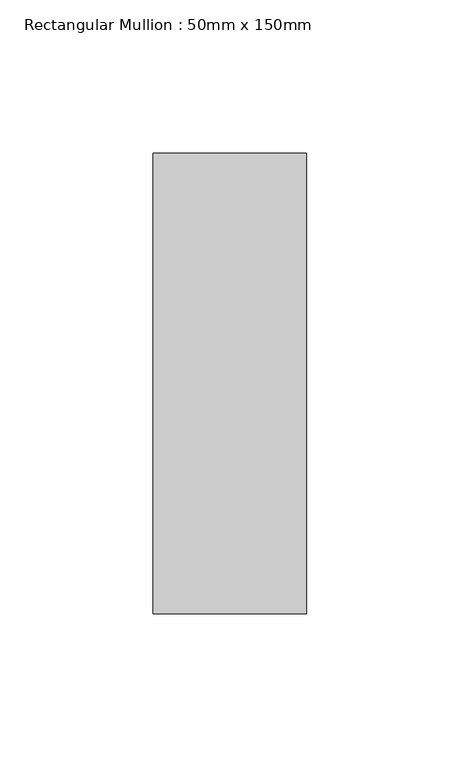
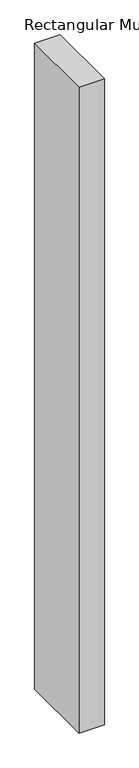
"""IFC4 building model written with IfcOpenShell, lengths in millimetres: member geometry, Rectangular Mullion : 50mm x 150mm."""

import ifcopenshell
import ifcopenshell.guid

model = None  # the IFC model being written
_history = None  # IfcOwnerHistory: only IFC2X3 demands one
_inside = {}  # id of a spatial element -> (the spatial element, [elements in it])
_under = {}  # id of a project, library or spatial element -> (it, [spatial elements below it])
_declared = {}  # id of a project -> (the project, [libraries it declares])
_typed = {}  # id of a type object -> (the type object, [elements of that type])
_made_of = {}  # id of a material, layer set ... -> (it, [elements and type objects made of it])


def new_model(schema):
    """Start an empty IFC model of exactly this schema.

    Asked for "IFC4X3", IfcOpenShell would pick the latest addendum, in which some entities
    have other attributes; the version numbers below select the first issue.
    IFC2X3 requires an IfcOwnerHistory on every rooted entity: one is made here for all.
    """
    global model, _history
    if schema == "IFC4X3":
        model = ifcopenshell.file(schema_version=(4, 3, 0, 0))
    else:
        model = ifcopenshell.file(schema=schema)
    _inside.clear()
    _under.clear()
    _declared.clear()
    _typed.clear()
    _made_of.clear()
    _history = None
    if model.schema == "IFC2X3":
        org = make("IfcOrganization", Name="unknown")
        user = make(
            "IfcPersonAndOrganization",
            ThePerson=make("IfcPerson", FamilyName="unknown"),
            TheOrganization=org,
        )
        app = make(
            "IfcApplication",
            ApplicationDeveloper=org,
            Version="unknown",
            ApplicationFullName="unknown",
            ApplicationIdentifier="unknown",
        )
        _history = make(
            "IfcOwnerHistory",
            OwningUser=user,
            OwningApplication=app,
            ChangeAction="ADDED",
            CreationDate=0,
        )
    return model


def make(cls, **values):
    """One entity of the class cls with the attributes given. An attribute that is None is left unset."""
    return model.create_entity(
        cls, **{name: value for name, value in values.items() if value is not None}
    )


def rooted(cls, **values):
    """An entity with a GlobalId (a new one), such as an element, a storey or a relation."""
    return make(cls, GlobalId=ifcopenshell.guid.new(), OwnerHistory=_history, **values)


def si_unit(unit_type, name, prefix=None):
    """IfcSIUnit, for example si_unit("LENGTHUNIT", "METRE", prefix="MILLI")."""
    return make("IfcSIUnit", UnitType=unit_type, Prefix=prefix, Name=name)


def assignment(units):
    """IfcUnitAssignment: the units of a project."""
    return None if units is None else make("IfcUnitAssignment", Units=units)


def point(xyz):
    """IfcCartesianPoint."""
    return None if xyz is None else make("IfcCartesianPoint", Coordinates=xyz)


def direction(xyz):
    """IfcDirection."""
    return None if xyz is None else make("IfcDirection", DirectionRatios=xyz)


def frame(location, z_axis=None, x_axis=None):
    """IfcAxis2Placement3D, a coordinate frame: its origin and axes. An axis left out is left unset."""
    return make(
        "IfcAxis2Placement3D",
        Location=point(location),
        Axis=direction(z_axis),
        RefDirection=direction(x_axis),
    )


def origin():
    """The frame at (0, 0, 0) with its axes left unset."""
    return frame((0.0, 0.0, 0.0))


def place(relative_to, where):
    """IfcLocalPlacement: puts the frame where relative to a parent placement (None: the world)."""
    return make(
        "IfcLocalPlacement", PlacementRelTo=relative_to, RelativePlacement=where
    )


def context(
    kind, dimensions, precision=None, world=None, true_north=None, identifier=None
):
    """IfcGeometricRepresentationContext, for example the 3D "Model" context."""
    return make(
        "IfcGeometricRepresentationContext",
        ContextIdentifier=identifier,
        ContextType=kind,
        CoordinateSpaceDimension=dimensions,
        Precision=precision,
        WorldCoordinateSystem=world,
        TrueNorth=true_north,
    )


def project(units=None, contexts=None):
    """IfcProject with its units and contexts."""
    return rooted(
        "IfcProject",
        Name="project",
        RepresentationContexts=contexts,
        UnitsInContext=assignment(units),
    )


def spatial(cls, under=None, at=None, **own):
    """A site, building, storey or space (cls), placed at a placement, below another one or the project."""
    s = rooted(cls, ObjectPlacement=at, **own)
    if under is not None:
        _under.setdefault(under.id(), (under, []))[1].append(s)
    return s


def polyline(points):
    """IfcPolyline through the points."""
    return make("IfcPolyline", Points=[point(p) for p in points])


def outline(outer, holes=None, kind="AREA"):
    """IfcArbitraryClosedProfileDef: a profile drawn as a closed curve; with holes, ...WithVoids."""
    if holes is None:
        return make("IfcArbitraryClosedProfileDef", ProfileType=kind, OuterCurve=outer)
    return make(
        "IfcArbitraryProfileDefWithVoids",
        ProfileType=kind,
        OuterCurve=outer,
        InnerCurves=holes,
    )


def extrude(swept, where, along, depth):
    """IfcExtrudedAreaSolid: the profile swept, set in the frame where, extruded along a direction by depth."""
    return make(
        "IfcExtrudedAreaSolid",
        SweptArea=swept,
        Position=where,
        ExtrudedDirection=direction(along),
        Depth=depth,
    )


def shape(context_of_items, identifier, shape_type, items):
    """IfcShapeRepresentation: the items that make up one representation, for example the "Body"."""
    return make(
        "IfcShapeRepresentation",
        ContextOfItems=context_of_items,
        RepresentationIdentifier=identifier,
        RepresentationType=shape_type,
        Items=items,
    )


def source(mapping_origin, context_of_items, identifier, shape_type, items):
    """IfcRepresentationMap: a shape defined once, which mapped items show again and again."""
    return make(
        "IfcRepresentationMap",
        MappingOrigin=mapping_origin,
        MappedRepresentation=shape(context_of_items, identifier, shape_type, items),
    )


def transform(
    local_origin,
    x_axis=None,
    y_axis=None,
    z_axis=None,
    scale=None,
    scale2=None,
    scale3=None,
    uniform=True,
):
    """IfcCartesianTransformationOperator3D, or its non-uniform kind. x_axis, y_axis, z_axis: its Axis1, 2, 3."""
    if uniform:
        return make(
            "IfcCartesianTransformationOperator3D",
            Axis1=direction(x_axis),
            Axis2=direction(y_axis),
            LocalOrigin=point(local_origin),
            Scale=scale,
            Axis3=direction(z_axis),
        )
    return make(
        "IfcCartesianTransformationOperator3DnonUniform",
        Axis1=direction(x_axis),
        Axis2=direction(y_axis),
        LocalOrigin=point(local_origin),
        Scale=scale,
        Axis3=direction(z_axis),
        Scale2=scale2,
        Scale3=scale3,
    )


def mapped(mapping_source, mapping_target):
    """IfcMappedItem: shows the shape of a source again, moved by a transform."""
    return make(
        "IfcMappedItem", MappingSource=mapping_source, MappingTarget=mapping_target
    )


def made_of(thing, what):
    """Note that an element or type object is made of a material, layer set ...; save() writes the relation."""
    if what is not None:
        _made_of.setdefault(what.id(), (what, []))[1].append(thing)
    return thing


def element(
    cls,
    number,
    at=None,
    inside=None,
    cuts=None,
    type_object=None,
    material=None,
    context=None,
    identifier="Body",
    shape_type=None,
    held_by="IfcProductDefinitionShape",
    body=None,
    shapes=None,
    **own,
):
    """One element of the class cls, such as IfcWall. Its Tag is "e" and its number.

    at: its placement. inside: the storey or other place that contains it. cuts: it is an
    opening in that element (IfcRelVoidsElement). A single representation is given by context,
    identifier, shape_type and body (its items); several are given by shapes. held_by: the class
    of the entity that holds the representations. save() writes the other relations.
    """
    e = rooted(cls, Tag="e%d" % number, ObjectPlacement=at, **own)
    if body is not None:
        shapes = [shape(context, identifier, shape_type, body)]
    if shapes is not None:
        e.Representation = make(held_by, Representations=shapes)
    if inside is not None:
        _inside.setdefault(inside.id(), (inside, []))[1].append(e)
    if cuts is not None:
        rooted(
            "IfcRelVoidsElement", RelatingBuildingElement=cuts, RelatedOpeningElement=e
        )
    if type_object is not None:
        _typed.setdefault(type_object.id(), (type_object, []))[1].append(e)
    return made_of(e, material)


def aggregate(whole, parts):
    """IfcRelAggregates: a whole, such as a stair, and the parts it consists of."""
    return rooted("IfcRelAggregates", RelatingObject=whole, RelatedObjects=parts)


def save(model, path):
    """Write the relations noted so far, then the file.

    IfcRelAggregates (storeys below a building ...), IfcRelContainedInSpatialStructure (elements
    in a storey), IfcRelDefinesByType, IfcRelAssociatesMaterial and IfcRelDeclares: one each for
    every whole, place, type object, material and project.
    """
    for whole, parts in _under.values():
        aggregate(whole, parts)
    for where, things in _inside.values():
        rooted(
            "IfcRelContainedInSpatialStructure",
            RelatedElements=things,
            RelatingStructure=where,
        )
    for kind, things in _typed.values():
        rooted("IfcRelDefinesByType", RelatedObjects=things, RelatingType=kind)
    for what, things in _made_of.values():
        rooted("IfcRelAssociatesMaterial", RelatedObjects=things, RelatingMaterial=what)
    for by, libraries in _declared.values():
        rooted("IfcRelDeclares", RelatingContext=by, RelatedDefinitions=libraries)
    model.write(path)


def rectangular_mullion_50mm_x_150mm_926b4069(model_context):
    return source(origin(), model_context, "Body", "SweptSolid", [
        extrude(outline(polyline([(0.0, 75.0), (0.0, -75.0), (-50.0, -75.0), (-50.0, 75.0), (0.0, 75.0)])), frame((0.0, 0.0, -1339.9999997), z_axis=(0.0, 0.0, 1.0), x_axis=(1.0, 0.0, 0.0)), (0.0, 0.0, 1.0), 1339.9999997),
    ])


if __name__ == "__main__":
    model = new_model("IFC4")
    model_context = context("Model", 3, world=origin())
    ifc_project = project(units=[si_unit("LENGTHUNIT", "METRE", prefix="MILLI")], contexts=[model_context])
    site = spatial("IfcSite", under=ifc_project)
    building = spatial("IfcBuilding", under=site)
    placement = place(None, origin())
    rectangular_mullion_50mm_x_150mm_shape = rectangular_mullion_50mm_x_150mm_926b4069(model_context)
    element("IfcMember", 1, ObjectType="Rectangular Mullion : 50mm x 150mm", at=placement, inside=building, context=model_context, shape_type="MappedRepresentation", body=[
        mapped(rectangular_mullion_50mm_x_150mm_shape, transform((0.0, 0.0, 0.0), x_axis=(1.0, 0.0, 0.0), y_axis=(0.0, 1.0, 0.0), z_axis=(0.0, 0.0, 1.0))),
    ])
    save(model, "model.ifc")

# Revit data of these elements
# Type "Rectangular Mullion : 50mm x 150mm"
#   built-in parameter 1007304 = 0.492126 (stored number, unit not read)
#   built-in parameter 1007301 = 0.082021 (stored number, unit not read)
#   built-in parameter 1007300 = 0.082021 (stored number, unit not read)
# Element 1 (IfcMember, "Rectangular Mullion : 50mm x 150mm")
#   Materials on its faces: "Aluminum"
# Materials
#   "Aluminum": class "Metal", colour RGB 244 244 244, transparency 0, Description = "Aluminum 6061", Cost = 0
